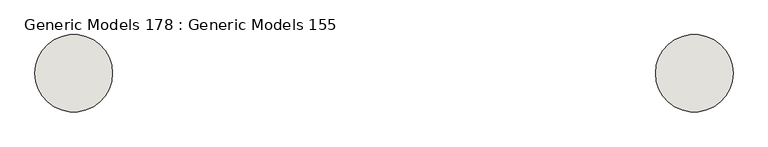
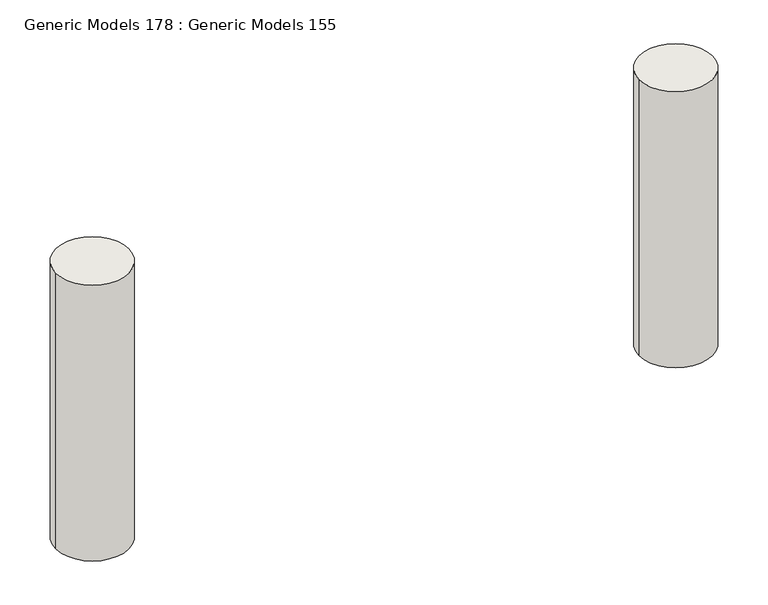
"""IFC4 building model written with IfcOpenShell, lengths in millimetres: wall geometry, Generic Models 178 : Generic Models 155."""

from ifc_helpers import new_model, si_unit, point, frame, frame_2d, origin, place, context, project, spatial, circle_curve, trimmed, segment, composite_curve, outline, extrude, source, transform, mapped, element, save


def generic_models_178_generic_models_155_a54ccf4c(model_context):
    return source(origin(), model_context, "Body", "SweptSolid", [
        extrude(outline(composite_curve([segment(trimmed(circle_curve(frame_2d((56595.9625, 458.7875)), 152.4), [point((56443.5625, 458.7875))], [point((56748.3625, 458.7875))], False, "CARTESIAN"), True, "CONTINUOUS"), segment(trimmed(circle_curve(frame_2d((56595.9625, 458.7875)), 152.4), [point((56748.3625, 458.7875))], [point((56443.5625, 458.7875))], False, "CARTESIAN"), True, "CONTINUOUS")], self_intersect=False)), frame((0.0, 0.0, -1219.2), z_axis=(0.0, 0.0, 1.0), x_axis=(1.0, 0.0, 0.0)), (0.0, 0.0, 1.0), 1219.2),
        extrude(outline(composite_curve([segment(trimmed(circle_curve(frame_2d((54157.5625, 458.7875)), 152.4), [point((54005.1625, 458.7875))], [point((54309.9625, 458.7875))], False, "CARTESIAN"), True, "CONTINUOUS"), segment(trimmed(circle_curve(frame_2d((54157.5625, 458.7875)), 152.4), [point((54309.9625, 458.7875))], [point((54005.1625, 458.7875))], False, "CARTESIAN"), True, "CONTINUOUS")], self_intersect=False)), frame((0.0, 0.0, -1219.2), z_axis=(0.0, 0.0, 1.0), x_axis=(1.0, 0.0, 0.0)), (0.0, 0.0, 1.0), 1219.2),
    ])


if __name__ == "__main__":
    model = new_model("IFC4")
    model_context = context("Model", 3, world=origin())
    ifc_project = project(units=[si_unit("LENGTHUNIT", "METRE", prefix="MILLI")], contexts=[model_context])
    site = spatial("IfcSite", under=ifc_project)
    building = spatial("IfcBuilding", under=site)
    placement = place(None, origin())
    generic_models_178_generic_models_155_shape = generic_models_178_generic_models_155_a54ccf4c(model_context)
    element("IfcWall", 1, ObjectType="Generic Models 178 : Generic Models 155", at=placement, inside=building, context=model_context, shape_type="MappedRepresentation", body=[
        mapped(generic_models_178_generic_models_155_shape, transform((0.0, 0.0, 0.0), x_axis=(1.0, 0.0, 0.0), y_axis=(0.0, 1.0, 0.0), z_axis=(0.0, 0.0, 1.0))),
    ])
    save(model, "model.ifc")

# Revit data of these elements
# Element 1 (IfcWall, "Generic Models 178 : Generic Models 155")
#   Materials on its faces: "CONCRETE (3000 PSI CONCRETE)"
# Materials
#   "CONCRETE (3000 PSI CONCRETE)": class "Concrete", colour RGB 192 192 192, transparency 0, Description = "Cast-in-place concrete", Cost = 0
